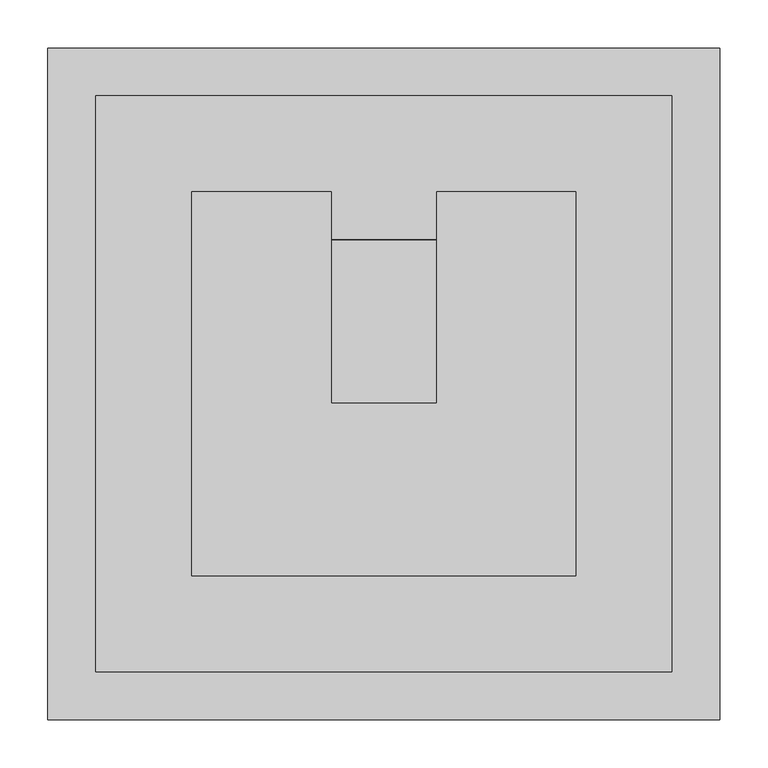
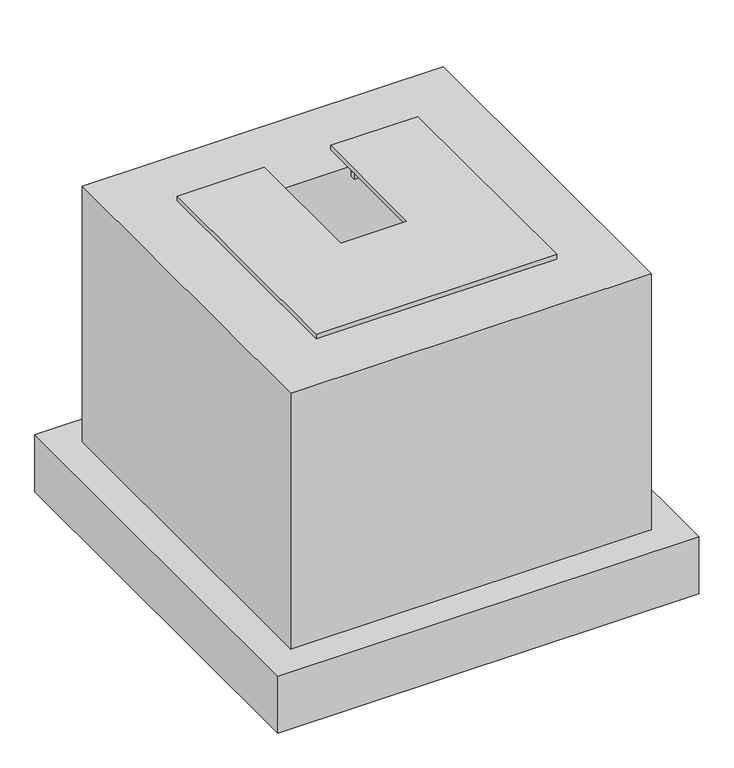
"""IFC4 building model written with IfcOpenShell, lengths in millimetres: proxy geometry, Catchpit : Rainwater Catchpit."""

from ifc_helpers import new_model, si_unit, frame, origin, origin_with_axes, place, context, project, spatial, polyline, outline, extrude, faceted_brep, source, transform, mapped, element, save


def generic_models_4b8b6a59(model_context):
    return source(origin(), model_context, "Body", "SolidModel", [
        extrude(outline(polyline([(-55.0, 140.0), (-55.0, 132.0), (-132.0, 132.0), (-132.0, -132.0), (132.0, -132.0), (132.0, 132.0), (55.0, 132.0), (55.0, 140.0), (140.0, 140.0), (140.0, -140.0), (-140.0, -140.0), (-140.0, 140.0), (-55.0, 140.0)])), frame((0.0, 0.0, -10.0), z_axis=(0.0, 0.0, 1.0), x_axis=(1.0, 0.0, 0.0)), (0.0, 0.0, 1.0), 10.0),
        extrude(outline(polyline([(-55.0, 200.0), (-55.0, -20.0), (55.0, -20.0), (55.0, 200.0), (200.0, 200.0), (200.0, -200.0), (-200.0, -200.0), (-200.0, 200.0), (-55.0, 200.0)])), origin_with_axes(), (0.0, 0.0, 1.0), 8.0),
        faceted_brep([(150.0, -150.0, -300.0), (150.0, 150.0, -300.0), (-150.0, 150.0, -300.0), (-150.0, -150.0, -300.0), (300.0, 300.0, -450.0), (300.0, -300.0, -450.0), (-300.0, -300.0, -450.0), (-300.0, 300.0, -450.0), (-300.0, 300.0, 0.0), (300.0, 300.0, 0.0), (-300.0, -300.0, 0.0), (300.0, -300.0, 0.0), (150.0, 150.0, 0.0), (150.0, -150.0, 0.0), (-150.0, -150.0, 0.0), (-150.0, 150.0, 0.0)], [[[0, 1, 2, 3]], [[4, 5, 6, 7]], [[4, 7, 8, 9]], [[8, 7, 6, 10]], [[10, 6, 5, 11]], [[11, 5, 4, 9]], [[9, 8, 10, 11], [12, 13, 14, 15]], [[13, 12, 1, 0]], [[14, 13, 0, 3]], [[15, 14, 3, 2]], [[12, 15, 2, 1]]]),
        extrude(outline(polyline([(350.0, 350.0), (350.0, -350.0), (-350.0, -350.0), (-350.0, 350.0), (350.0, 350.0)])), frame((0.0, 0.0, -550.0), z_axis=(0.0, 0.0, 1.0), x_axis=(1.0, 0.0, 0.0)), (0.0, 0.0, 1.0), 100.0),
    ])


if __name__ == "__main__":
    model = new_model("IFC4")
    model_context = context("Model", 3, world=origin())
    ifc_project = project(units=[si_unit("LENGTHUNIT", "METRE", prefix="MILLI")], contexts=[model_context])
    site = spatial("IfcSite", under=ifc_project)
    building = spatial("IfcBuilding", under=site)
    placement = place(None, origin())
    generic_models_shape = generic_models_4b8b6a59(model_context)
    element("IfcBuildingElementProxy", 1, Name="Catchpit : Rainwater Catchpit", ObjectType="Catchpit : Rainwater Catchpit", at=placement, inside=building, context=model_context, shape_type="MappedRepresentation", body=[
        mapped(generic_models_shape, transform((0.0, 0.0, 0.0), x_axis=(1.0, 0.0, 0.0), y_axis=(0.0, 1.0, 0.0), z_axis=(0.0, 0.0, 1.0))),
    ])
    save(model, "model.ifc")

# Revit data of these elements
# Type "Catchpit : Rainwater Catchpit"
#   Width = 300 mm
#   Wall Thk = 150 mm
#   Slab Thk = 150 mm
#   Length = 300 mm
#   Lean Thk = 100 mm
#   Lean Edge = 50 mm
#   Height = 300 mm
#   FB Thk = 8 mm
#   FB Length = 10 mm
#   Cutting Width = 110 mm
#   Cutting Length = 220 mm
#   Chk'd PL Thk = 8 mm
#   Structure Material = none
#   Lean_Material = none
#   CHK`D = none
#   Default Elevation = 0
